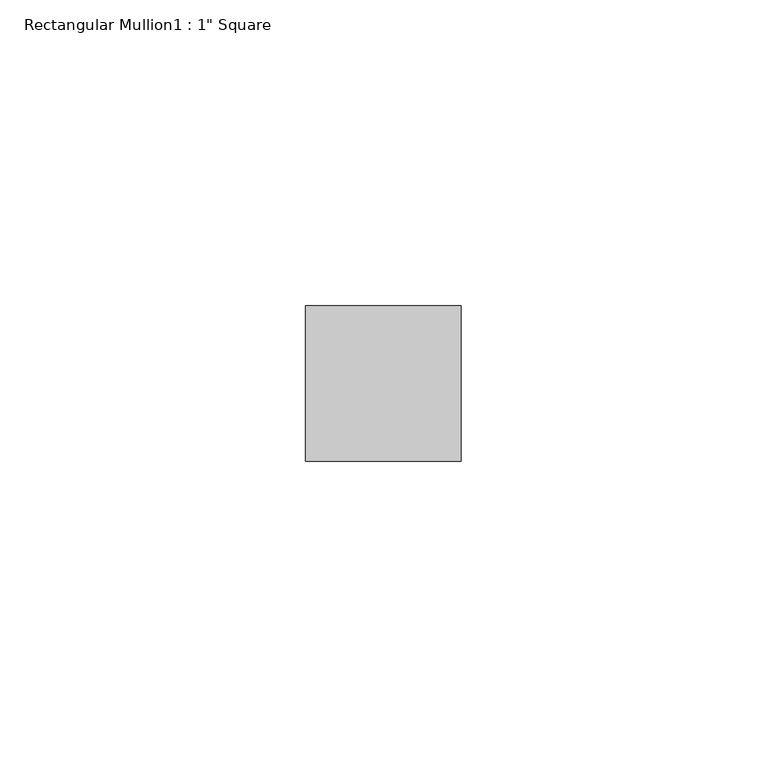
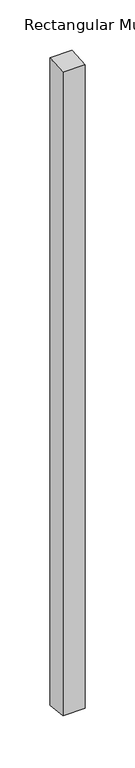
"""IFC4 building model written with IfcOpenShell, lengths in millimetres: member geometry."""

from ifc_helpers import new_model, si_unit, frame, origin, place, context, project, spatial, polyline, outline, extrude, source, transform, mapped, element, save


def member_7d7b18c4(model_context):
    return source(origin(), model_context, "Body", "SweptSolid", [
        extrude(outline(polyline([(-44.45, -4.2341647), (-19.05, -1.814642), (-19.05, -788.2125933), (-44.45, -785.7930706), (-44.45, -4.2341647)])), frame((-12.7, 0.0, 0.0), z_axis=(1.0, 0.0, 0.0), x_axis=(0.0, 1.0, 0.0)), (0.0, 0.0, 1.0), 25.4),
    ])


if __name__ == "__main__":
    model = new_model("IFC4")
    model_context = context("Model", 3, world=origin())
    ifc_project = project(units=[si_unit("LENGTHUNIT", "METRE", prefix="MILLI")], contexts=[model_context])
    site = spatial("IfcSite", under=ifc_project)
    building = spatial("IfcBuilding", under=site)
    placement = place(None, origin())
    member_shape = member_7d7b18c4(model_context)
    element("IfcMember", 1, ObjectType="Rectangular Mullion1 : 1\" Square", at=placement, inside=building, context=model_context, shape_type="MappedRepresentation", body=[
        mapped(member_shape, transform((0.0, 0.0, 0.0), x_axis=(1.0, 0.0, 0.0), y_axis=(0.0, 1.0, 0.0), z_axis=(0.0, 0.0, 1.0))),
    ])
    save(model, "model.ifc")

# Revit data of these elements
# Type "Rectangular Mullion1 : 1\" Square"
#   built-in parameter 1007351 = 0.104167 (stored number, unit not read)
#   built-in parameter 1007304 = 0.0833333 (stored number, unit not read)
#   built-in parameter 1007301 = 0.0416667 (stored number, unit not read)
#   built-in parameter 1007300 = 0.0416667 (stored number, unit not read)
